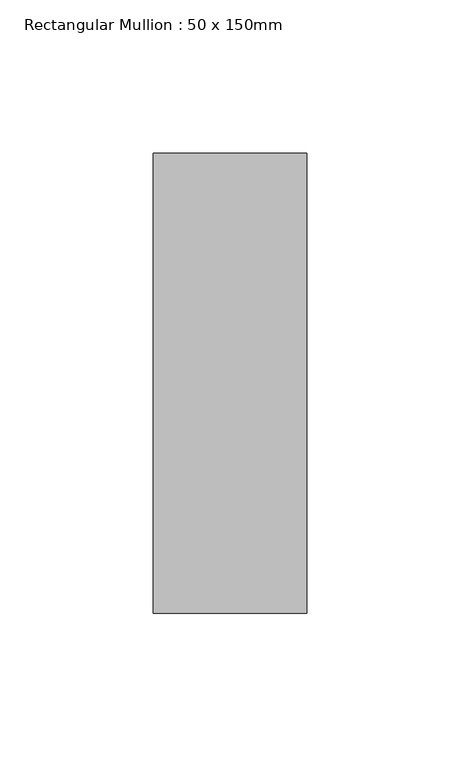
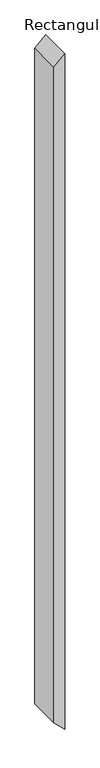
"""IFC4 building model written with IfcOpenShell, lengths in millimetres: member geometry, Rectangular Mullion : 50 x 150mm."""

from ifc_helpers import new_model, si_unit, frame, origin, place, context, project, spatial, polyline, outline, extrude, source, transform, mapped, element, save


def rectangular_mullion_50_x_150mm_5afc71bb(model_context):
    return source(origin(), model_context, "Body", "SweptSolid", [
        extrude(outline(polyline([(0.0, 0.0), (-47.0734921, -50.0), (-3194.7760444, -50.0), (-3244.7760444, 0.0), (0.0, 0.0)])), frame((0.0, -75.0, 0.0), z_axis=(0.0, 1.0, 0.0), x_axis=(0.0, 0.0, 1.0)), (0.0, 0.0, 1.0), 150.0),
    ])


if __name__ == "__main__":
    model = new_model("IFC4")
    model_context = context("Model", 3, world=origin())
    ifc_project = project(units=[si_unit("LENGTHUNIT", "METRE", prefix="MILLI")], contexts=[model_context])
    site = spatial("IfcSite", under=ifc_project)
    building = spatial("IfcBuilding", under=site)
    placement = place(None, origin())
    rectangular_mullion_50_x_150mm_shape = rectangular_mullion_50_x_150mm_5afc71bb(model_context)
    element("IfcMember", 1, ObjectType="Rectangular Mullion : 50 x 150mm", at=placement, inside=building, context=model_context, shape_type="MappedRepresentation", body=[
        mapped(rectangular_mullion_50_x_150mm_shape, transform((0.0, 0.0, 0.0), x_axis=(1.0, 0.0, 0.0), y_axis=(0.0, 1.0, 0.0), z_axis=(0.0, 0.0, 1.0))),
    ])
    save(model, "model.ifc")

# Revit data of these elements
# Type "Rectangular Mullion : 50 x 150mm"
#   built-in parameter 1007304 = 0.492126 (stored number, unit not read)
#   built-in parameter 1007301 = 0.082021 (stored number, unit not read)
#   built-in parameter 1007300 = 0.082021 (stored number, unit not read)
# Element 1 (IfcMember, "Rectangular Mullion : 50 x 150mm")
#   Materials on its faces: "Metal - Aluminium"
# Materials
#   "Metal - Aluminium": class "Metal", colour RGB 247 247 247, transparency 0
